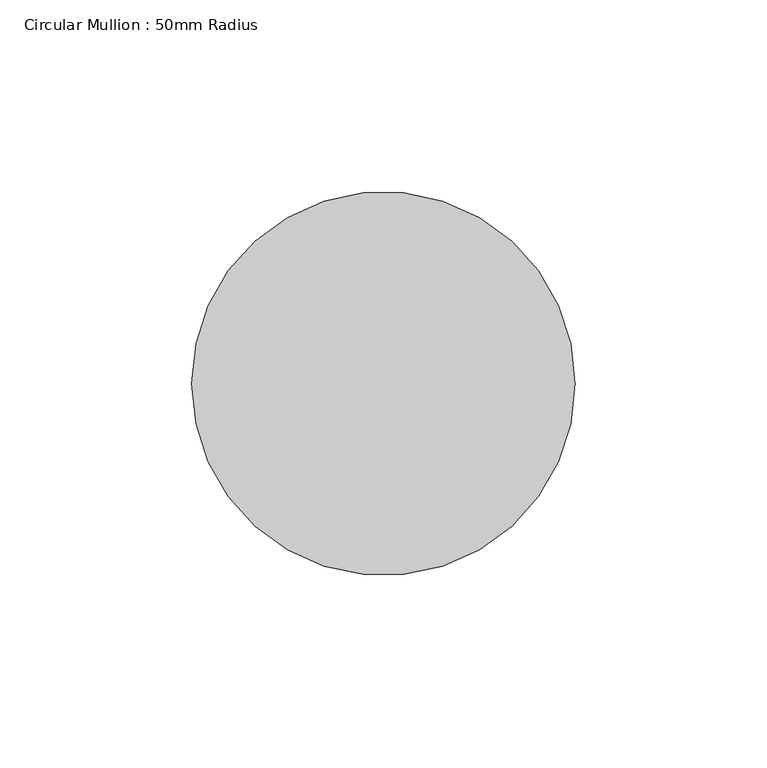
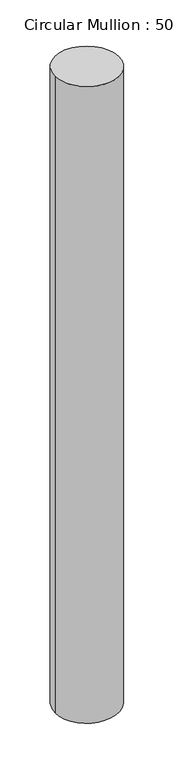
"""IFC4 building model written with IfcOpenShell, lengths in millimetres: member geometry, Circular Mullion : 50mm Radius."""

from ifc_helpers import new_model, si_unit, frame, origin, place, context, project, spatial, ellipse_curve, source, transform, mapped, element, save
from ifc_brep_helpers import plane_surface, cylinder_surface, advanced_brep


def circular_mullion_50mm_radius_4a483d66(model_context):
    return source(origin(), model_context, "Body", "AdvancedBrep", [
        advanced_brep(
        [(-100.0, 0.0, 1.6916568), (0.0, 0.0, 0.0), (0.0, 0.0, -1052.121026), (-100.0, 0.0, -1053.8813371)],
        [
            (0, 1, ellipse_curve(frame((-50.0, 0.0, 0.8458284), z_axis=(-0.016910021034786775, -0.02208830545715375, -0.9996130040924012), x_axis=(-0.6076449356244492, -0.7937214814786068, 0.027818016632478244)), 50.0193573, 50.0)),
            (1, 2),
            (2, 3, ellipse_curve(frame((-50.0, 0.0, -1053.0011816), z_axis=(-0.017595734888021724, -0.02298400257162447, 0.9995809750788268), x_axis=(0.6076254658217821, 0.7936960495204703, 0.028946057770645975)), 50.02096, 50.0)),
            (3, 0),
            (1, 0, ellipse_curve(frame((-50.0, 0.0, 0.8458284), z_axis=(-0.016910021034786775, -0.02208830545715375, -0.9996130040924012), x_axis=(-0.6076449356244492, -0.7937214814786068, 0.027818016632478244)), 50.0193573, 50.0)),
            (3, 2, ellipse_curve(frame((-50.0, 0.0, -1053.0011816), z_axis=(-0.017595734888021724, -0.02298400257162447, 0.9995809750788268), x_axis=(0.6076254658217821, 0.7936960495204703, 0.028946057770645975)), 50.02096, 50.0)),
        ],
        [
            cylinder_surface(frame((-50.0, 0.0, 0.0), z_axis=(0.0, 0.0, 1.0), x_axis=(1.0, 0.0, 0.0)), 50.0),
            plane_surface(frame((-242.0199683, 185.2818797, 0.0), z_axis=(0.016910021034786775, 0.02208830545715375, 0.9996130040924012), x_axis=(0.6076449356244499, 0.7937214814786059, -0.027818016632489444))),
            plane_surface(frame((-242.0199683, 185.2818797, -1052.121026), z_axis=(0.017595734888021724, 0.02298400257162447, -0.9995809750788268), x_axis=(0.607625465821782, 0.7936960495204701, 0.02894605777065307))),
        ],
        [
            (0, [[1, 2, 3, 4]]),
            (0, [[5, -4, 6, -2]]),
            (1, [[-1, -5]]),
            (2, [[-6, -3]]),
        ],
    ),
    ])


if __name__ == "__main__":
    model = new_model("IFC4")
    model_context = context("Model", 3, world=origin())
    ifc_project = project(units=[si_unit("LENGTHUNIT", "METRE", prefix="MILLI")], contexts=[model_context])
    site = spatial("IfcSite", under=ifc_project)
    building = spatial("IfcBuilding", under=site)
    placement = place(None, origin())
    circular_mullion_50mm_radius_shape = circular_mullion_50mm_radius_4a483d66(model_context)
    element("IfcMember", 1, ObjectType="Circular Mullion : 50mm Radius", at=placement, inside=building, context=model_context, shape_type="MappedRepresentation", body=[
        mapped(circular_mullion_50mm_radius_shape, transform((0.0, 0.0, 0.0), x_axis=(1.0, 0.0, 0.0), y_axis=(0.0, 1.0, 0.0), z_axis=(0.0, 0.0, 1.0))),
    ])
    save(model, "model.ifc")

# Revit data of these elements
# Type "Circular Mullion : 50mm Radius"
#   built-in parameter 1007350 = 0.164042 (stored number, unit not read)
# Element 1 (IfcMember, "Circular Mullion : 50mm Radius")
#   Materials on its faces: "Aluminium"
# Materials
#   "Aluminium": class "Metal", colour RGB 247 247 247, transparency 0, Description = "Aluminium 6061", Cost = 0
